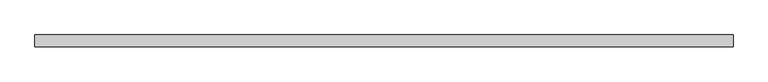
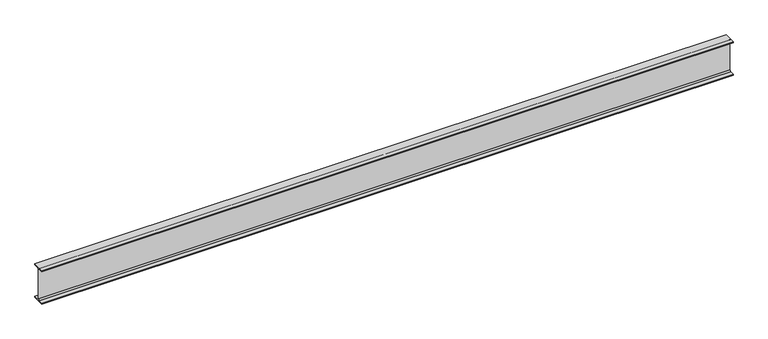
"""IFC4 building model written with IfcOpenShell, lengths in millimetres: beam geometry, Steel Framing_H_KS : H_SB_AR_S02_H-600x200x11x17_SRB2."""

from ifc_helpers import new_model, si_unit, point, frame, frame_2d, origin, place, context, project, spatial, polyline, circle_curve, trimmed, segment, composite_curve, outline, extrude, source, transform, mapped, element, save


def beam_0d7a42ae(model_context):
    return source(origin(), model_context, "Body", "SweptSolid", [
        extrude(outline(composite_curve([segment(polyline([(100.0, -283.0), (100.0, -300.0), (-100.0, -300.0), (-100.0, -283.0), (-27.5, -283.0)]), True, "CONTINUOUS"), segment(trimmed(circle_curve(frame_2d((-27.5, -261.0)), 22.0), [point((-27.5, -283.0))], [point((-5.5, -261.0))], True, "CARTESIAN"), True, "CONTINUOUS"), segment(polyline([(-5.5, -261.0), (-5.5, 261.0)]), True, "CONTINUOUS"), segment(trimmed(circle_curve(frame_2d((-27.5, 261.0)), 22.0), [point((-5.5, 261.0))], [point((-27.5, 283.0))], True, "CARTESIAN"), True, "CONTINUOUS"), segment(polyline([(-27.5, 283.0), (-100.0, 283.0), (-100.0, 300.0), (100.0, 300.0), (100.0, 283.0), (27.5, 283.0)]), True, "CONTINUOUS"), segment(trimmed(circle_curve(frame_2d((27.5, 261.0)), 22.0), [point((27.5, 283.0))], [point((5.5, 261.0))], True, "CARTESIAN"), True, "CONTINUOUS"), segment(polyline([(5.5, 261.0), (5.5, -261.0)]), True, "CONTINUOUS"), segment(trimmed(circle_curve(frame_2d((27.5, -261.0)), 22.0), [point((5.5, -261.0))], [point((27.5, -283.0))], True, "CARTESIAN"), True, "CONTINUOUS"), segment(polyline([(27.5, -283.0), (100.0, -283.0)]), True, "CONTINUOUS")], self_intersect=False)), frame((-5912.3, 0.0, 0.0), z_axis=(1.0, 0.0, 0.0), x_axis=(0.0, 1.0, 0.0)), (0.0, 0.0, 1.0), 11749.6),
    ])


if __name__ == "__main__":
    model = new_model("IFC4")
    model_context = context("Model", 3, world=origin())
    ifc_project = project(units=[si_unit("LENGTHUNIT", "METRE", prefix="MILLI")], contexts=[model_context])
    site = spatial("IfcSite", under=ifc_project)
    building = spatial("IfcBuilding", under=site)
    placement = place(None, origin())
    beam_shape = beam_0d7a42ae(model_context)
    element("IfcBeam", 1, ObjectType="Steel Framing_H_KS : H_SB_AR_S02_H-600x200x11x17_SRB2", at=placement, inside=building, context=model_context, shape_type="MappedRepresentation", body=[
        mapped(beam_shape, transform((0.0, 0.0, 0.0), x_axis=(1.0, 0.0, 0.0), y_axis=(0.0, 1.0, 0.0), z_axis=(0.0, 0.0, 1.0))),
    ])
    save(model, "model.ifc")

# Revit data of these elements
# Type "Steel Framing_H_KS : H_SB_AR_S02_H-600x200x11x17_SRB2"
#   Type Comments = "MAIN"
#   Type Mark = "SRB2"
#   H_SectionID = "H-600x200x11x17"
#   H_Ratio for Additional Steel Plate = 0.2
#   Width = 20.0 cm
#   Web Thickness = 1.1 cm
#   Web Fillet = 2.2 cm
#   Warping Constant = 1930000.0 cm⁶
#   Torsional Moment of Inertia = 91.3724 cm⁴
#   Section Area = 134.4 cm²
#   Plastic Modulus weak axis = 361.0 cm³
#   Plastic Modulus strong axis = 2980.0 cm³
#   Perimeter = 1.94 m²/m
#   Nominal Weight = 106.00 kgf/m
#   Moment of Inertia weak axis = 2280.00 cm⁴
#   Moment of Inertia strong axis = 77600.00 cm⁴
#   Height = 60.0 cm
#   Flange Thickness = 1.7 cm
#   Elastic Modulus weak axis = 228.0 cm³
#   Elastic Modulus strong axis = 2590.0 cm³
#   Centroid Vertical = 30.0 cm
#   Centroid Horizontal = 10.0 cm
#   Bolt Spacing = 8.89 cm
#   Length [instance default] = 1500 mm
#   Structural Material [instance default] = Steel, 45-345
#   Section Name Key = ""
#   Assembly Code = ""
# Element 1 (IfcBeam, "Steel Framing_H_KS : H_SB_AR_S02_H-600x200x11x17_SRB2")
#   Materials on its faces: "Steel, 45-345"
# Materials
#   "Steel, 45-345": class "Metal", colour RGB 189 187 185, transparency 0, Description = "Steel 345 MPa", Cost = 0
